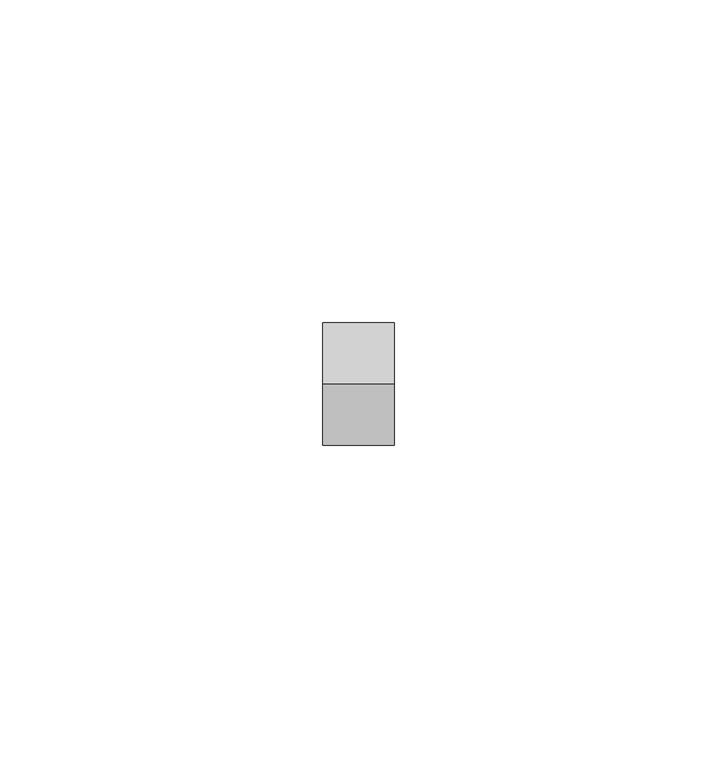
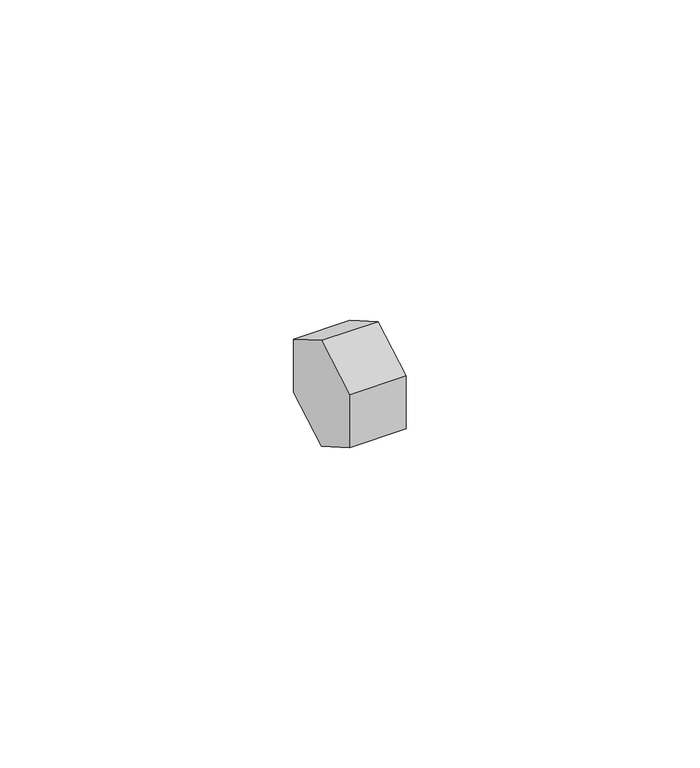
"""IFC4 building model written with IfcOpenShell, lengths in millimetres: proxy geometry, Generic Models 7:Generic Models 1:8:Generic Models 1:8 : Generic Models 7:Generic Models 1:337419:55 : Generic Models 7:Generic Models 1:8:Generic Models 1:8 : Generic Models 7:Generic Models 1:337419:315935."""

import ifcopenshell
import ifcopenshell.guid

model = None  # the IFC model being written
_history = None  # IfcOwnerHistory: only IFC2X3 demands one
_inside = {}  # id of a spatial element -> (the spatial element, [elements in it])
_under = {}  # id of a project, library or spatial element -> (it, [spatial elements below it])
_declared = {}  # id of a project -> (the project, [libraries it declares])
_typed = {}  # id of a type object -> (the type object, [elements of that type])
_made_of = {}  # id of a material, layer set ... -> (it, [elements and type objects made of it])


def new_model(schema):
    """Start an empty IFC model of exactly this schema.

    Asked for "IFC4X3", IfcOpenShell would pick the latest addendum, in which some entities
    have other attributes; the version numbers below select the first issue.
    IFC2X3 requires an IfcOwnerHistory on every rooted entity: one is made here for all.
    """
    global model, _history
    if schema == "IFC4X3":
        model = ifcopenshell.file(schema_version=(4, 3, 0, 0))
    else:
        model = ifcopenshell.file(schema=schema)
    _inside.clear()
    _under.clear()
    _declared.clear()
    _typed.clear()
    _made_of.clear()
    _history = None
    if model.schema == "IFC2X3":
        org = make("IfcOrganization", Name="unknown")
        user = make(
            "IfcPersonAndOrganization",
            ThePerson=make("IfcPerson", FamilyName="unknown"),
            TheOrganization=org,
        )
        app = make(
            "IfcApplication",
            ApplicationDeveloper=org,
            Version="unknown",
            ApplicationFullName="unknown",
            ApplicationIdentifier="unknown",
        )
        _history = make(
            "IfcOwnerHistory",
            OwningUser=user,
            OwningApplication=app,
            ChangeAction="ADDED",
            CreationDate=0,
        )
    return model


def make(cls, **values):
    """One entity of the class cls with the attributes given. An attribute that is None is left unset."""
    return model.create_entity(
        cls, **{name: value for name, value in values.items() if value is not None}
    )


def rooted(cls, **values):
    """An entity with a GlobalId (a new one), such as an element, a storey or a relation."""
    return make(cls, GlobalId=ifcopenshell.guid.new(), OwnerHistory=_history, **values)


def si_unit(unit_type, name, prefix=None):
    """IfcSIUnit, for example si_unit("LENGTHUNIT", "METRE", prefix="MILLI")."""
    return make("IfcSIUnit", UnitType=unit_type, Prefix=prefix, Name=name)


def assignment(units):
    """IfcUnitAssignment: the units of a project."""
    return None if units is None else make("IfcUnitAssignment", Units=units)


def point(xyz):
    """IfcCartesianPoint."""
    return None if xyz is None else make("IfcCartesianPoint", Coordinates=xyz)


def direction(xyz):
    """IfcDirection."""
    return None if xyz is None else make("IfcDirection", DirectionRatios=xyz)


def frame(location, z_axis=None, x_axis=None):
    """IfcAxis2Placement3D, a coordinate frame: its origin and axes. An axis left out is left unset."""
    return make(
        "IfcAxis2Placement3D",
        Location=point(location),
        Axis=direction(z_axis),
        RefDirection=direction(x_axis),
    )


def origin():
    """The frame at (0, 0, 0) with its axes left unset."""
    return frame((0.0, 0.0, 0.0))


def place(relative_to, where):
    """IfcLocalPlacement: puts the frame where relative to a parent placement (None: the world)."""
    return make(
        "IfcLocalPlacement", PlacementRelTo=relative_to, RelativePlacement=where
    )


def context(
    kind, dimensions, precision=None, world=None, true_north=None, identifier=None
):
    """IfcGeometricRepresentationContext, for example the 3D "Model" context."""
    return make(
        "IfcGeometricRepresentationContext",
        ContextIdentifier=identifier,
        ContextType=kind,
        CoordinateSpaceDimension=dimensions,
        Precision=precision,
        WorldCoordinateSystem=world,
        TrueNorth=true_north,
    )


def project(units=None, contexts=None):
    """IfcProject with its units and contexts."""
    return rooted(
        "IfcProject",
        Name="project",
        RepresentationContexts=contexts,
        UnitsInContext=assignment(units),
    )


def spatial(cls, under=None, at=None, **own):
    """A site, building, storey or space (cls), placed at a placement, below another one or the project."""
    s = rooted(cls, ObjectPlacement=at, **own)
    if under is not None:
        _under.setdefault(under.id(), (under, []))[1].append(s)
    return s


def polyline(points):
    """IfcPolyline through the points."""
    return make("IfcPolyline", Points=[point(p) for p in points])


def outline(outer, holes=None, kind="AREA"):
    """IfcArbitraryClosedProfileDef: a profile drawn as a closed curve; with holes, ...WithVoids."""
    if holes is None:
        return make("IfcArbitraryClosedProfileDef", ProfileType=kind, OuterCurve=outer)
    return make(
        "IfcArbitraryProfileDefWithVoids",
        ProfileType=kind,
        OuterCurve=outer,
        InnerCurves=holes,
    )


def extrude(swept, where, along, depth):
    """IfcExtrudedAreaSolid: the profile swept, set in the frame where, extruded along a direction by depth."""
    return make(
        "IfcExtrudedAreaSolid",
        SweptArea=swept,
        Position=where,
        ExtrudedDirection=direction(along),
        Depth=depth,
    )


def shape(context_of_items, identifier, shape_type, items):
    """IfcShapeRepresentation: the items that make up one representation, for example the "Body"."""
    return make(
        "IfcShapeRepresentation",
        ContextOfItems=context_of_items,
        RepresentationIdentifier=identifier,
        RepresentationType=shape_type,
        Items=items,
    )


def source(mapping_origin, context_of_items, identifier, shape_type, items):
    """IfcRepresentationMap: a shape defined once, which mapped items show again and again."""
    return make(
        "IfcRepresentationMap",
        MappingOrigin=mapping_origin,
        MappedRepresentation=shape(context_of_items, identifier, shape_type, items),
    )


def transform(
    local_origin,
    x_axis=None,
    y_axis=None,
    z_axis=None,
    scale=None,
    scale2=None,
    scale3=None,
    uniform=True,
):
    """IfcCartesianTransformationOperator3D, or its non-uniform kind. x_axis, y_axis, z_axis: its Axis1, 2, 3."""
    if uniform:
        return make(
            "IfcCartesianTransformationOperator3D",
            Axis1=direction(x_axis),
            Axis2=direction(y_axis),
            LocalOrigin=point(local_origin),
            Scale=scale,
            Axis3=direction(z_axis),
        )
    return make(
        "IfcCartesianTransformationOperator3DnonUniform",
        Axis1=direction(x_axis),
        Axis2=direction(y_axis),
        LocalOrigin=point(local_origin),
        Scale=scale,
        Axis3=direction(z_axis),
        Scale2=scale2,
        Scale3=scale3,
    )


def mapped(mapping_source, mapping_target):
    """IfcMappedItem: shows the shape of a source again, moved by a transform."""
    return make(
        "IfcMappedItem", MappingSource=mapping_source, MappingTarget=mapping_target
    )


def made_of(thing, what):
    """Note that an element or type object is made of a material, layer set ...; save() writes the relation."""
    if what is not None:
        _made_of.setdefault(what.id(), (what, []))[1].append(thing)
    return thing


def element(
    cls,
    number,
    at=None,
    inside=None,
    cuts=None,
    type_object=None,
    material=None,
    context=None,
    identifier="Body",
    shape_type=None,
    held_by="IfcProductDefinitionShape",
    body=None,
    shapes=None,
    **own,
):
    """One element of the class cls, such as IfcWall. Its Tag is "e" and its number.

    at: its placement. inside: the storey or other place that contains it. cuts: it is an
    opening in that element (IfcRelVoidsElement). A single representation is given by context,
    identifier, shape_type and body (its items); several are given by shapes. held_by: the class
    of the entity that holds the representations. save() writes the other relations.
    """
    e = rooted(cls, Tag="e%d" % number, ObjectPlacement=at, **own)
    if body is not None:
        shapes = [shape(context, identifier, shape_type, body)]
    if shapes is not None:
        e.Representation = make(held_by, Representations=shapes)
    if inside is not None:
        _inside.setdefault(inside.id(), (inside, []))[1].append(e)
    if cuts is not None:
        rooted(
            "IfcRelVoidsElement", RelatingBuildingElement=cuts, RelatedOpeningElement=e
        )
    if type_object is not None:
        _typed.setdefault(type_object.id(), (type_object, []))[1].append(e)
    return made_of(e, material)


def aggregate(whole, parts):
    """IfcRelAggregates: a whole, such as a stair, and the parts it consists of."""
    return rooted("IfcRelAggregates", RelatingObject=whole, RelatedObjects=parts)


def save(model, path):
    """Write the relations noted so far, then the file.

    IfcRelAggregates (storeys below a building ...), IfcRelContainedInSpatialStructure (elements
    in a storey), IfcRelDefinesByType, IfcRelAssociatesMaterial and IfcRelDeclares: one each for
    every whole, place, type object, material and project.
    """
    for whole, parts in _under.values():
        aggregate(whole, parts)
    for where, things in _inside.values():
        rooted(
            "IfcRelContainedInSpatialStructure",
            RelatedElements=things,
            RelatingStructure=where,
        )
    for kind, things in _typed.values():
        rooted("IfcRelDefinesByType", RelatedObjects=things, RelatingType=kind)
    for what, things in _made_of.values():
        rooted("IfcRelAssociatesMaterial", RelatedObjects=things, RelatingMaterial=what)
    for by, libraries in _declared.values():
        rooted("IfcRelDeclares", RelatingContext=by, RelatedDefinitions=libraries)
    model.write(path)


def generic_models_d1ff193a(model_context):
    return source(origin(), model_context, "Body", "SweptSolid", [
        extrude(outline(polyline([(-564919.104849, 8833.512141), (-564928.629849, 8839.0114023), (-564928.629849, 8850.009925), (-564919.104849, 8855.5091863), (-564909.579849, 8850.009925), (-564909.579849, 8839.0114023), (-564919.104849, 8833.512141)])), frame((593654.1476618, 0.0, 0.0), z_axis=(1.0, 0.0, 0.0), x_axis=(0.0, 1.0, 0.0)), (0.0, 0.0, 1.0), 11.1125),
    ])


if __name__ == "__main__":
    model = new_model("IFC4")
    model_context = context("Model", 3, world=origin())
    ifc_project = project(units=[si_unit("LENGTHUNIT", "METRE", prefix="MILLI")], contexts=[model_context])
    site = spatial("IfcSite", under=ifc_project)
    building = spatial("IfcBuilding", under=site)
    placement = place(None, origin())
    generic_models_shape = generic_models_d1ff193a(model_context)
    element("IfcBuildingElementProxy", 1, Name="Generic Models 7:Generic Models 1:8:Generic Models 1:8 : Generic Models 7:Generic Models 1:337419:55 : Generic Models 7:Generic Models 1:8:Generic Models 1:8 : Generic Models 7:Generic Models 1:337419:315935", ObjectType="Generic Models 7:Generic Models 1:8:Generic Models 1:8 : Generic Models 7:Generic Models 1:337419:55 : Generic Models 7:Generic Models 1:8:Generic Models 1:8 : Generic Models 7:Generic Models 1:337419:315935", at=placement, inside=building, context=model_context, shape_type="MappedRepresentation", body=[
        mapped(generic_models_shape, transform((0.0, 0.0, 0.0), x_axis=(1.0, 0.0, 0.0), y_axis=(0.0, 1.0, 0.0), z_axis=(0.0, 0.0, 1.0))),
    ])
    save(model, "model.ifc")

# Revit data of these elements
# Type "Generic Models 7:Generic Models 1:8:Generic Models 1:8 : Generic Models 7:Generic Models 1:337419:55 : Generic Models 7:Generic Models 1:8:Generic Models 1:8 : Generic Models 7:Generic Models 1:337419:315935"
#   NameOverride = "Generic Models 7:Generic Models 1:8:Generic Models 1:8 : Generic Models 7:Generic Models 1:337419:315935"
#   ObjectTypeOverride = "Generic Models 1:8 : Generic Models 7:Generic Models 1:337419"
#   Reference = "Generic Models 1"
#   Tag = "315935"
# Element 1 (IfcBuildingElementProxy, "Generic Models 7:Generic Models 1:8:Generic Models 1:8 : Generic Models 7:Generic Models 1:337419:55 : Generic Models 7:Generic Models 1:8:Generic Models 1:8 : Generic Models 7:Generic Models 1:337419:315935")
#   Materials on its faces: "1/2\" THRU BOLTS"
# Materials
#   "1/2\" THRU BOLTS": class "Generic", colour RGB 120 120 120, transparency 0, Cost = 0
